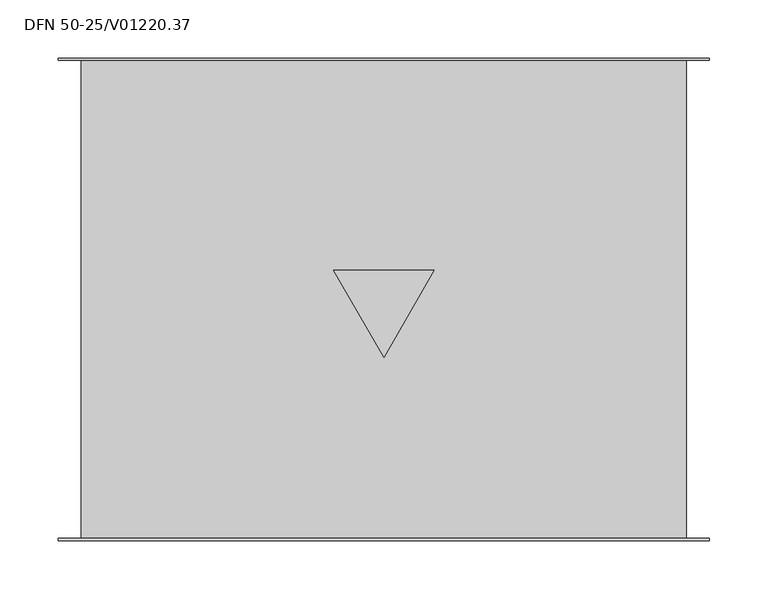
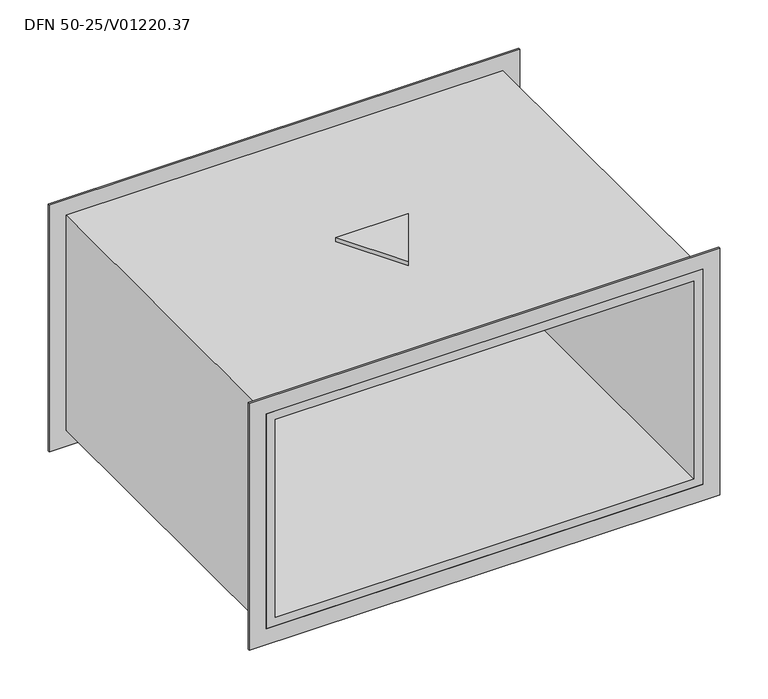
"""IFC4 building model written with IfcOpenShell, lengths in millimetres: proxy geometry, Вентилятор канальный DFN : DFN 50-25/V01220.37."""

from ifc_helpers import new_model, si_unit, frame, origin, place, context, project, spatial, polyline, outline, extrude, source, transform, mapped, element, save


def dfn_50_25_v01220_37_296fb525(model_context):
    return source(origin(), model_context, "Body", "SweptSolid", [
        extrude(outline(polyline([(43.3012702, 25.0), (0.0, -50.0), (-43.3012702, 25.0), (43.3012702, 25.0)])), frame((0.0, 0.0, 136.0), z_axis=(0.0, 0.0, 1.0), x_axis=(1.0, 0.0, 0.0)), (0.0, 0.0, 1.0), 5.0),
        extrude(outline(polyline([(156.0, 281.0), (156.0, -281.0), (-156.0, -281.0), (-156.0, 281.0), (156.0, 281.0)]), holes=[polyline([(-136.0, 261.0), (-136.0, -261.0), (136.0, -261.0), (136.0, 261.0), (-136.0, 261.0)])]), frame((0.0, 206.0, 0.0), z_axis=(0.0, 1.0, 0.0), x_axis=(0.0, 0.0, 1.0)), (0.0, 0.0, 1.0), 2.0),
        extrude(outline(polyline([(156.0, -281.0), (-156.0, -281.0), (-156.0, 281.0), (156.0, 281.0), (156.0, -281.0)]), holes=[polyline([(136.0, 261.0), (-136.0, 261.0), (-136.0, -261.0), (136.0, -261.0), (136.0, 261.0)])]), frame((0.0, -208.0, 0.0), z_axis=(0.0, 1.0, 0.0), x_axis=(0.0, 0.0, 1.0)), (0.0, 0.0, 1.0), 2.0),
        extrude(outline(polyline([(136.0, 261.0), (136.0, -261.0), (-136.0, -261.0), (-136.0, 261.0), (136.0, 261.0)]), holes=[polyline([(125.0, 250.0), (-125.0, 250.0), (-125.0, -250.0), (125.0, -250.0), (125.0, 250.0)])]), frame((0.0, -208.0, 0.0), z_axis=(0.0, 1.0, 0.0), x_axis=(0.0, 0.0, 1.0)), (0.0, 0.0, 1.0), 416.0),
    ])


if __name__ == "__main__":
    model = new_model("IFC4")
    model_context = context("Model", 3, world=origin())
    ifc_project = project(units=[si_unit("LENGTHUNIT", "METRE", prefix="MILLI")], contexts=[model_context])
    site = spatial("IfcSite", under=ifc_project)
    building = spatial("IfcBuilding", under=site)
    placement = place(None, origin())
    dfn_50_25_v01220_37_shape = dfn_50_25_v01220_37_296fb525(model_context)
    element("IfcBuildingElementProxy", 1, Name="Вентилятор канальный DFN : DFN 50-25/V01220.37", ObjectType="Вентилятор канальный DFN : DFN 50-25/V01220.37", at=placement, inside=building, context=model_context, shape_type="MappedRepresentation", body=[
        mapped(dfn_50_25_v01220_37_shape, transform((0.0, 0.0, 0.0), x_axis=(1.0, 0.0, 0.0), y_axis=(0.0, 1.0, 0.0), z_axis=(0.0, 0.0, 1.0))),
    ])
    save(model, "model.ifc")

# Revit data of these elements
# Type "Вентилятор канальный DFN : DFN 50-25/V01220.37"
#   Manufacturer = "WAER"
#   URL = "https://waer-air.com/"
#   ADSK_Система_Имя [instance default] = ""
#   ADSK_Наименование краткое = "DFN 50-25/V01220.37"
#   ADSK_Наименование = "Венилятор канальный DFN 50-25/V01220.37"
#   ADSK_Масса_Текст = "26"
#   ADSK_Марка = ""
#   ADSK_Код изделия = ""
#   ADSK_Завод-изготовитель = "WAER"
#   ADSK_Единица измерения = "шт."
#   Ширина_В = 522 mm
#   Высота_Г = 272 mm
#   ADSK_Ток = 1.01 A
#   ADSK_Расход воздуха = 0 m³/h
#   ADSK_Размер_Ширина = 500 mm
#   ADSK_Размер_Длина = 416 mm
#   ADSK_Размер_Высота = 250 mm
#   ADSK_Потеря давления воздуха = 0.0 Pa
#   ADSK_Полная мощность = 383.8 VA
#   ADSK_Номинальная мощность = 0.37 W
#   ADSK_Напряжение = 380 V
#   ADSK_Масса = 26
#   ADSK_Количество = 1
#   ADSK_Количество фаз = 3
#   ADSK_Классификация нагрузок = ОВК
#   Default Elevation = 0
#   Keynote = ""
